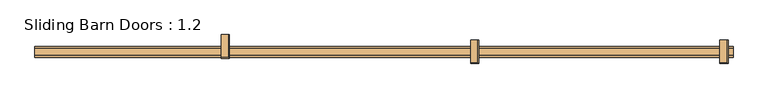
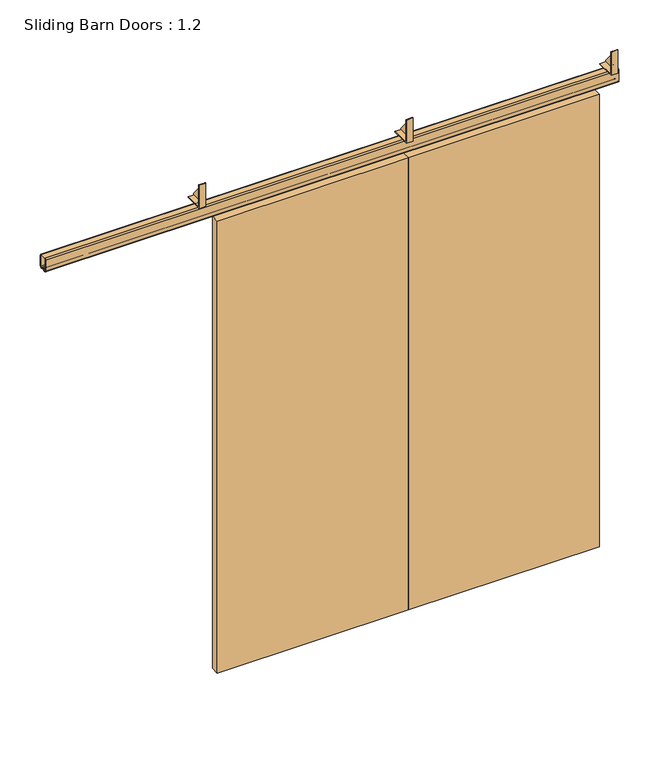
"""IFC4 building model written with IfcOpenShell, lengths in millimetres: door geometry, Sliding Barn Doors : 1.2."""

import ifcopenshell
import ifcopenshell.guid

model = None  # the IFC model being written
_history = None  # IfcOwnerHistory: only IFC2X3 demands one
_inside = {}  # id of a spatial element -> (the spatial element, [elements in it])
_under = {}  # id of a project, library or spatial element -> (it, [spatial elements below it])
_declared = {}  # id of a project -> (the project, [libraries it declares])
_typed = {}  # id of a type object -> (the type object, [elements of that type])
_made_of = {}  # id of a material, layer set ... -> (it, [elements and type objects made of it])


def new_model(schema):
    """Start an empty IFC model of exactly this schema.

    Asked for "IFC4X3", IfcOpenShell would pick the latest addendum, in which some entities
    have other attributes; the version numbers below select the first issue.
    IFC2X3 requires an IfcOwnerHistory on every rooted entity: one is made here for all.
    """
    global model, _history
    if schema == "IFC4X3":
        model = ifcopenshell.file(schema_version=(4, 3, 0, 0))
    else:
        model = ifcopenshell.file(schema=schema)
    _inside.clear()
    _under.clear()
    _declared.clear()
    _typed.clear()
    _made_of.clear()
    _history = None
    if model.schema == "IFC2X3":
        org = make("IfcOrganization", Name="unknown")
        user = make(
            "IfcPersonAndOrganization",
            ThePerson=make("IfcPerson", FamilyName="unknown"),
            TheOrganization=org,
        )
        app = make(
            "IfcApplication",
            ApplicationDeveloper=org,
            Version="unknown",
            ApplicationFullName="unknown",
            ApplicationIdentifier="unknown",
        )
        _history = make(
            "IfcOwnerHistory",
            OwningUser=user,
            OwningApplication=app,
            ChangeAction="ADDED",
            CreationDate=0,
        )
    return model


def make(cls, **values):
    """One entity of the class cls with the attributes given. An attribute that is None is left unset."""
    return model.create_entity(
        cls, **{name: value for name, value in values.items() if value is not None}
    )


def rooted(cls, **values):
    """An entity with a GlobalId (a new one), such as an element, a storey or a relation."""
    return make(cls, GlobalId=ifcopenshell.guid.new(), OwnerHistory=_history, **values)


def si_unit(unit_type, name, prefix=None):
    """IfcSIUnit, for example si_unit("LENGTHUNIT", "METRE", prefix="MILLI")."""
    return make("IfcSIUnit", UnitType=unit_type, Prefix=prefix, Name=name)


def assignment(units):
    """IfcUnitAssignment: the units of a project."""
    return None if units is None else make("IfcUnitAssignment", Units=units)


def point(xyz):
    """IfcCartesianPoint."""
    return None if xyz is None else make("IfcCartesianPoint", Coordinates=xyz)


def direction(xyz):
    """IfcDirection."""
    return None if xyz is None else make("IfcDirection", DirectionRatios=xyz)


def frame(location, z_axis=None, x_axis=None):
    """IfcAxis2Placement3D, a coordinate frame: its origin and axes. An axis left out is left unset."""
    return make(
        "IfcAxis2Placement3D",
        Location=point(location),
        Axis=direction(z_axis),
        RefDirection=direction(x_axis),
    )


def frame_2d(location, x_axis=None):
    """IfcAxis2Placement2D, a coordinate frame in the plane: its origin and x axis."""
    return make(
        "IfcAxis2Placement2D", Location=point(location), RefDirection=direction(x_axis)
    )


def origin():
    """The frame at (0, 0, 0) with its axes left unset."""
    return frame((0.0, 0.0, 0.0))


def place(relative_to, where):
    """IfcLocalPlacement: puts the frame where relative to a parent placement (None: the world)."""
    return make(
        "IfcLocalPlacement", PlacementRelTo=relative_to, RelativePlacement=where
    )


def context(
    kind, dimensions, precision=None, world=None, true_north=None, identifier=None
):
    """IfcGeometricRepresentationContext, for example the 3D "Model" context."""
    return make(
        "IfcGeometricRepresentationContext",
        ContextIdentifier=identifier,
        ContextType=kind,
        CoordinateSpaceDimension=dimensions,
        Precision=precision,
        WorldCoordinateSystem=world,
        TrueNorth=true_north,
    )


def project(units=None, contexts=None):
    """IfcProject with its units and contexts."""
    return rooted(
        "IfcProject",
        Name="project",
        RepresentationContexts=contexts,
        UnitsInContext=assignment(units),
    )


def spatial(cls, under=None, at=None, **own):
    """A site, building, storey or space (cls), placed at a placement, below another one or the project."""
    s = rooted(cls, ObjectPlacement=at, **own)
    if under is not None:
        _under.setdefault(under.id(), (under, []))[1].append(s)
    return s


def polyline(points):
    """IfcPolyline through the points."""
    return make("IfcPolyline", Points=[point(p) for p in points])


def circle_curve(where, radius):
    """IfcCircle in the frame where."""
    return make("IfcCircle", Position=where, Radius=radius)


def trimmed(basis, trim1, trim2, sense, master):
    """IfcTrimmedCurve: the piece of a basis curve between two trims."""
    return make(
        "IfcTrimmedCurve",
        BasisCurve=basis,
        Trim1=trim1,
        Trim2=trim2,
        SenseAgreement=sense,
        MasterRepresentation=master,
    )


def segment(curve, same_sense, transition):
    """IfcCompositeCurveSegment."""
    return make(
        "IfcCompositeCurveSegment",
        Transition=transition,
        SameSense=same_sense,
        ParentCurve=curve,
    )


def composite_curve(segments, self_intersect=None):
    """IfcCompositeCurve: segments joined end to end."""
    return make("IfcCompositeCurve", Segments=segments, SelfIntersect=self_intersect)


def outline(outer, holes=None, kind="AREA"):
    """IfcArbitraryClosedProfileDef: a profile drawn as a closed curve; with holes, ...WithVoids."""
    if holes is None:
        return make("IfcArbitraryClosedProfileDef", ProfileType=kind, OuterCurve=outer)
    return make(
        "IfcArbitraryProfileDefWithVoids",
        ProfileType=kind,
        OuterCurve=outer,
        InnerCurves=holes,
    )


def extrude(swept, where, along, depth):
    """IfcExtrudedAreaSolid: the profile swept, set in the frame where, extruded along a direction by depth."""
    return make(
        "IfcExtrudedAreaSolid",
        SweptArea=swept,
        Position=where,
        ExtrudedDirection=direction(along),
        Depth=depth,
    )


def shape(context_of_items, identifier, shape_type, items):
    """IfcShapeRepresentation: the items that make up one representation, for example the "Body"."""
    return make(
        "IfcShapeRepresentation",
        ContextOfItems=context_of_items,
        RepresentationIdentifier=identifier,
        RepresentationType=shape_type,
        Items=items,
    )


def source(mapping_origin, context_of_items, identifier, shape_type, items):
    """IfcRepresentationMap: a shape defined once, which mapped items show again and again."""
    return make(
        "IfcRepresentationMap",
        MappingOrigin=mapping_origin,
        MappedRepresentation=shape(context_of_items, identifier, shape_type, items),
    )


def transform(
    local_origin,
    x_axis=None,
    y_axis=None,
    z_axis=None,
    scale=None,
    scale2=None,
    scale3=None,
    uniform=True,
):
    """IfcCartesianTransformationOperator3D, or its non-uniform kind. x_axis, y_axis, z_axis: its Axis1, 2, 3."""
    if uniform:
        return make(
            "IfcCartesianTransformationOperator3D",
            Axis1=direction(x_axis),
            Axis2=direction(y_axis),
            LocalOrigin=point(local_origin),
            Scale=scale,
            Axis3=direction(z_axis),
        )
    return make(
        "IfcCartesianTransformationOperator3DnonUniform",
        Axis1=direction(x_axis),
        Axis2=direction(y_axis),
        LocalOrigin=point(local_origin),
        Scale=scale,
        Axis3=direction(z_axis),
        Scale2=scale2,
        Scale3=scale3,
    )


def mapped(mapping_source, mapping_target):
    """IfcMappedItem: shows the shape of a source again, moved by a transform."""
    return make(
        "IfcMappedItem", MappingSource=mapping_source, MappingTarget=mapping_target
    )


def made_of(thing, what):
    """Note that an element or type object is made of a material, layer set ...; save() writes the relation."""
    if what is not None:
        _made_of.setdefault(what.id(), (what, []))[1].append(thing)
    return thing


def element(
    cls,
    number,
    at=None,
    inside=None,
    cuts=None,
    type_object=None,
    material=None,
    context=None,
    identifier="Body",
    shape_type=None,
    held_by="IfcProductDefinitionShape",
    body=None,
    shapes=None,
    **own,
):
    """One element of the class cls, such as IfcWall. Its Tag is "e" and its number.

    at: its placement. inside: the storey or other place that contains it. cuts: it is an
    opening in that element (IfcRelVoidsElement). A single representation is given by context,
    identifier, shape_type and body (its items); several are given by shapes. held_by: the class
    of the entity that holds the representations. save() writes the other relations.
    """
    e = rooted(cls, Tag="e%d" % number, ObjectPlacement=at, **own)
    if body is not None:
        shapes = [shape(context, identifier, shape_type, body)]
    if shapes is not None:
        e.Representation = make(held_by, Representations=shapes)
    if inside is not None:
        _inside.setdefault(inside.id(), (inside, []))[1].append(e)
    if cuts is not None:
        rooted(
            "IfcRelVoidsElement", RelatingBuildingElement=cuts, RelatedOpeningElement=e
        )
    if type_object is not None:
        _typed.setdefault(type_object.id(), (type_object, []))[1].append(e)
    return made_of(e, material)


def aggregate(whole, parts):
    """IfcRelAggregates: a whole, such as a stair, and the parts it consists of."""
    return rooted("IfcRelAggregates", RelatingObject=whole, RelatedObjects=parts)


def save(model, path):
    """Write the relations noted so far, then the file.

    IfcRelAggregates (storeys below a building ...), IfcRelContainedInSpatialStructure (elements
    in a storey), IfcRelDefinesByType, IfcRelAssociatesMaterial and IfcRelDeclares: one each for
    every whole, place, type object, material and project.
    """
    for whole, parts in _under.values():
        aggregate(whole, parts)
    for where, things in _inside.values():
        rooted(
            "IfcRelContainedInSpatialStructure",
            RelatedElements=things,
            RelatingStructure=where,
        )
    for kind, things in _typed.values():
        rooted("IfcRelDefinesByType", RelatedObjects=things, RelatingType=kind)
    for what, things in _made_of.values():
        rooted("IfcRelAssociatesMaterial", RelatedObjects=things, RelatingMaterial=what)
    for by, libraries in _declared.values():
        rooted("IfcRelDeclares", RelatingContext=by, RelatedDefinitions=libraries)
    model.write(path)


def sliding_barn_doors_1_2_d088c784(model_context):
    return source(origin(), model_context, "Body", "SweptSolid", [
        extrude(outline(polyline([(158.75, 2152.65), (158.75, 2146.3), (79.375, 2146.3), (79.375, 2247.773), (158.75, 2152.65)])), frame((-1354.9808594, 0.0, 0.0), z_axis=(1.0, 0.0, 0.0), x_axis=(0.0, 1.0, 0.0)), (0.0, 0.0, 1.0), 3.175),
        extrude(outline(polyline([(76.2, 2143.125), (76.2, 2247.773), (79.375, 2247.773), (79.375, 2146.3), (158.75, 2146.3), (158.75, 2143.125), (76.2, 2143.125)])), frame((-1380.2816406, 0.0, 0.0), z_axis=(1.0, 0.0, 0.0), x_axis=(0.0, 1.0, 0.0)), (0.0, 0.0, 1.0), 28.4757812),
        extrude(outline(polyline([(139.7, 2152.65), (139.7, 2146.3), (60.325, 2146.3), (60.325, 2247.773), (139.7, 2152.65)])), frame((-484.2371094, 0.0, 0.0), z_axis=(1.0, 0.0, 0.0), x_axis=(0.0, 1.0, 0.0)), (0.0, 0.0, 1.0), 3.175),
        extrude(outline(polyline([(57.15, 2143.125), (57.15, 2247.773), (60.325, 2247.773), (60.325, 2146.3), (139.7, 2146.3), (139.7, 2143.125), (57.15, 2143.125)])), frame((-509.5378906, 0.0, 0.0), z_axis=(1.0, 0.0, 0.0), x_axis=(0.0, 1.0, 0.0)), (0.0, 0.0, 1.0), 28.4757813),
        extrude(outline(polyline([(139.7, 2152.65), (139.7, 2146.3), (60.325, 2146.3), (60.325, 2247.773), (139.7, 2152.65)])), frame((386.5066406, 0.0, 0.0), z_axis=(1.0, 0.0, 0.0), x_axis=(0.0, 1.0, 0.0)), (0.0, 0.0, 1.0), 3.175),
        extrude(outline(polyline([(57.15, 2143.125), (57.15, 2247.773), (60.325, 2247.773), (60.325, 2146.3), (139.7, 2146.3), (139.7, 2143.125), (57.15, 2143.125)])), frame((361.2058594, 0.0, 0.0), z_axis=(1.0, 0.0, 0.0), x_axis=(0.0, 1.0, 0.0)), (0.0, 0.0, 1.0), 28.4757813),
        extrude(outline(polyline([(-1199.61025, 117.475), (-1148.30225, 117.475), (-1148.30225, 114.3), (-1199.61025, 114.3), (-1199.61025, 117.475)])), frame((0.0, 0.0, 1889.252), z_axis=(0.0, 0.0, 1.0), x_axis=(1.0, 0.0, 0.0)), (0.0, 0.0, 1.0), 168.148),
        extrude(outline(polyline([(-640.81025, 117.475), (-589.50225, 117.475), (-589.50225, 114.3), (-640.81025, 114.3), (-640.81025, 117.475)])), frame((0.0, 0.0, 1889.252), z_axis=(0.0, 0.0, 1.0), x_axis=(1.0, 0.0, 0.0)), (0.0, 0.0, 1.0), 168.148),
        extrude(outline(polyline([(-386.81025, 117.475), (-335.50225, 117.475), (-335.50225, 114.3), (-386.81025, 114.3), (-386.81025, 117.475)])), frame((0.0, 0.0, 1889.252), z_axis=(0.0, 0.0, 1.0), x_axis=(1.0, 0.0, 0.0)), (0.0, 0.0, 1.0), 168.148),
        extrude(outline(polyline([(171.98975, 117.475), (223.29775, 117.475), (223.29775, 114.3), (171.98975, 114.3), (171.98975, 117.475)])), frame((0.0, 0.0, 1889.252), z_axis=(0.0, 0.0, 1.0), x_axis=(1.0, 0.0, 0.0)), (0.0, 0.0, 1.0), 168.148),
        extrude(outline(polyline([(-1300.95625, 114.3), (-488.15625, 114.3), (-488.15625, 79.375), (-1300.95625, 79.375), (-1300.95625, 114.3)])), frame((0.0, 0.0, 25.4), z_axis=(0.0, 0.0, 1.0), x_axis=(1.0, 0.0, 0.0)), (0.0, 0.0, 1.0), 2032.0),
        extrude(outline(polyline([(-488.15625, 114.3), (324.64375, 114.3), (324.64375, 79.375), (-488.15625, 79.375), (-488.15625, 114.3)])), frame((0.0, 0.0, 25.4), z_axis=(0.0, 0.0, 1.0), x_axis=(1.0, 0.0, 0.0)), (0.0, 0.0, 1.0), 2032.0),
        extrude(outline(composite_curve([segment(polyline([(85.725, 2143.125), (111.252, 2143.125)]), True, "CONTINUOUS"), segment(trimmed(circle_curve(frame_2d((111.252, 2136.775)), 6.35), [point((111.252, 2143.125))], [point((117.602, 2136.775))], False, "CARTESIAN"), True, "CONTINUOUS"), segment(polyline([(117.602, 2136.775), (117.602, 2088.515)]), True, "CONTINUOUS"), segment(trimmed(circle_curve(frame_2d((111.252, 2088.515)), 6.35), [point((117.602, 2088.515))], [point((111.252, 2082.165))], False, "CARTESIAN"), True, "CONTINUOUS"), segment(polyline([(111.252, 2082.165), (105.8433147, 2082.165)]), True, "CONTINUOUS"), segment(trimmed(circle_curve(frame_2d((105.8433147, 2083.7525)), 1.5875), [point((105.8433147, 2082.165))], [point((104.2849816, 2083.4495907))], False, "CARTESIAN"), True, "CONTINUOUS"), segment(polyline([(104.2849816, 2083.4495907), (102.8594659, 2090.7832331), (104.3756029, 2090.7832331), (105.7615251, 2083.6532812), (111.252, 2083.6532812)]), True, "CONTINUOUS"), segment(trimmed(circle_curve(frame_2d((111.252, 2088.515)), 4.8617187), [point((111.252, 2083.6532812))], [point((116.1137188, 2088.515))], True, "CARTESIAN"), True, "CONTINUOUS"), segment(polyline([(116.1137188, 2088.515), (116.1137188, 2136.775)]), True, "CONTINUOUS"), segment(trimmed(circle_curve(frame_2d((111.252, 2136.775)), 4.8617187), [point((116.1137188, 2136.775))], [point((111.252, 2141.6367187))], True, "CARTESIAN"), True, "CONTINUOUS"), segment(polyline([(111.252, 2141.6367187), (85.725, 2141.6367187)]), True, "CONTINUOUS"), segment(trimmed(circle_curve(frame_2d((85.725, 2136.775)), 4.8617187), [point((85.725, 2141.6367187))], [point((80.8632813, 2136.775))], True, "CARTESIAN"), True, "CONTINUOUS"), segment(polyline([(80.8632813, 2136.775), (80.8632813, 2088.515)]), True, "CONTINUOUS"), segment(trimmed(circle_curve(frame_2d((85.725, 2088.515)), 4.8617187), [point((80.8632813, 2088.515))], [point((85.725, 2083.6532812))], True, "CARTESIAN"), True, "CONTINUOUS"), segment(polyline([(85.725, 2083.6532812), (91.2154749, 2083.6532812), (92.6013971, 2090.7832331), (94.1175341, 2090.7832331), (92.6920184, 2083.4495907)]), True, "CONTINUOUS"), segment(trimmed(circle_curve(frame_2d((91.1336853, 2083.7525)), 1.5875), [point((92.6920184, 2083.4495907))], [point((91.1336853, 2082.165))], False, "CARTESIAN"), True, "CONTINUOUS"), segment(polyline([(91.1336853, 2082.165), (85.725, 2082.165)]), True, "CONTINUOUS"), segment(trimmed(circle_curve(frame_2d((85.725, 2088.515)), 6.35), [point((85.725, 2082.165))], [point((79.375, 2088.515))], False, "CARTESIAN"), True, "CONTINUOUS"), segment(polyline([(79.375, 2088.515), (79.375, 2136.775)]), True, "CONTINUOUS"), segment(trimmed(circle_curve(frame_2d((85.725, 2136.775)), 6.35), [point((79.375, 2136.775))], [point((85.725, 2143.125))], False, "CARTESIAN"), True, "CONTINUOUS")], self_intersect=False)), frame((-2031.20625, 0.0, 0.0), z_axis=(1.0, 0.0, 0.0), x_axis=(0.0, 1.0, 0.0)), (0.0, 0.0, 1.0), 2438.4),
    ])


if __name__ == "__main__":
    model = new_model("IFC4")
    model_context = context("Model", 3, world=origin())
    ifc_project = project(units=[si_unit("LENGTHUNIT", "METRE", prefix="MILLI")], contexts=[model_context])
    site = spatial("IfcSite", under=ifc_project)
    building = spatial("IfcBuilding", under=site)
    placement = place(None, origin())
    sliding_barn_doors_1_2_shape = sliding_barn_doors_1_2_d088c784(model_context)
    element("IfcDoor", 1, ObjectType="Sliding Barn Doors : 1.2", at=placement, inside=building, context=model_context, shape_type="MappedRepresentation", body=[
        mapped(sliding_barn_doors_1_2_shape, transform((0.0, 0.0, 0.0), x_axis=(1.0, 0.0, 0.0), y_axis=(0.0, 1.0, 0.0), z_axis=(0.0, 0.0, 1.0))),
    ])
    save(model, "model.ifc")

# Revit data of these elements
# Type "Sliding Barn Doors : 1.2"
#   Type Mark = "44"
#   Analytic Construction = "<None>"
#   rail_overlap_left = 0' - 5 1/4"
#   rail_length = 8' - 0"
#   overlap_left = 0' - 2"
#   overlap = 0' - 0"
#   bracket_right = 3' - 7"
#   bracket_left = 0' - 4"
#   Thickness = 0' - 1 3/8"
#   Panel Width = 2' - 8"
#   Panel Height = 6' - 8"
#   Gap 2 = 0' - 0 1/2"
#   Gap 1 = 0' - 0 7/8"
#   Frame Projection Ext. = 0' - 1"
#   Frame Projection Int. = 0' - 1"
#   Frame Width = 0' - 3"
#   Height = 6' - 4"
#   Width = 1' - 9 9/16"
#   Bracket_offset = 0' - 5"
#   Door_4 = no
#   Door_3 = no
#   Hardware Material = Metal - Aluminum
#   Door Material = Closet_1
#   Function = (empty or 0)
#   Wall Closure = (empty or 0)
# Element 1 (IfcDoor, "Sliding Barn Doors : 1.2")
#   Materials on its faces: "Metal - Aluminum", "Closet_1"
# Materials
#   "Metal - Aluminum": class "Metal", colour RGB 247 247 247, transparency 0
#   "Closet_1": class "Paint", colour RGB 58 62 47, transparency 0, Cost = 0
